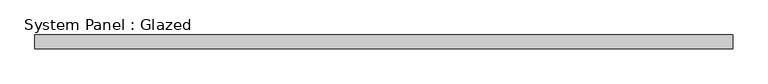
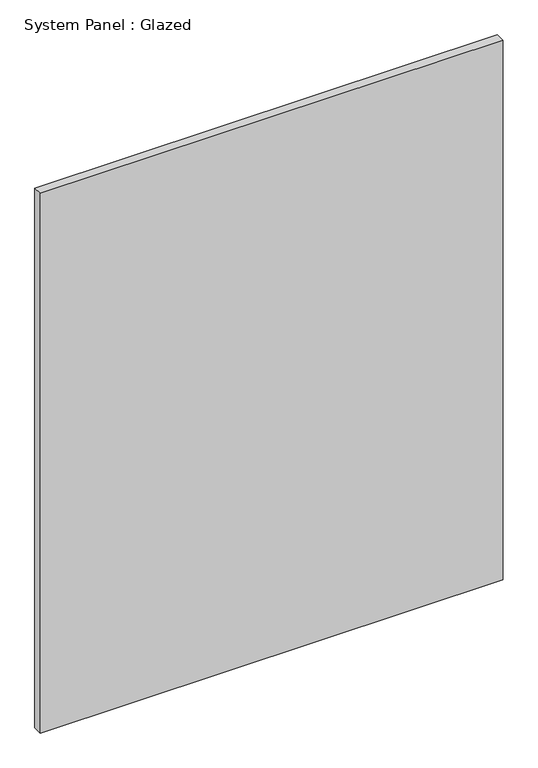
"""IFC4 building model written with IfcOpenShell, lengths in millimetres: plate geometry, System Panel : Glazed."""

from ifc_helpers import new_model, si_unit, origin, origin_with_axes, place, context, project, spatial, polyline, outline, extrude, source, transform, mapped, element, save


def system_panel_glazed_79b5039f(model_context):
    return source(origin(), model_context, "Body", "SweptSolid", [
        extrude(outline(polyline([(633.0541355, 24.5), (-633.0541355, 24.5), (-633.0541355, 49.5), (633.0541355, 49.5), (633.0541355, 24.5)])), origin_with_axes(), (0.0, 0.0, 1.0), 1560.0991456),
    ])


if __name__ == "__main__":
    model = new_model("IFC4")
    model_context = context("Model", 3, world=origin())
    ifc_project = project(units=[si_unit("LENGTHUNIT", "METRE", prefix="MILLI")], contexts=[model_context])
    site = spatial("IfcSite", under=ifc_project)
    building = spatial("IfcBuilding", under=site)
    placement = place(None, origin())
    system_panel_glazed_shape = system_panel_glazed_79b5039f(model_context)
    element("IfcPlate", 1, ObjectType="System Panel : Glazed", at=placement, inside=building, context=model_context, shape_type="MappedRepresentation", body=[
        mapped(system_panel_glazed_shape, transform((0.0, 0.0, 0.0), x_axis=(1.0, 0.0, 0.0), y_axis=(0.0, 1.0, 0.0), z_axis=(0.0, 0.0, 1.0))),
    ])
    save(model, "model.ifc")

# Revit data of these elements
# Type "System Panel : Glazed"
#   Construction Type Id = "GSP4R"
#   Analytic Construction = "1/8 in Pilkington single glazing"
#   Visual Light Transmittance = 0.9
#   Solar Heat Gain Coefficient = 0.86
#   Heat Transfer Coefficient (U) = 6.7069 W/(m²·K)
#   Define Thermal Properties by = 1
# Element 1 (IfcPlate, "System Panel : Glazed")
#   Materials on its faces: "Glass"
# Materials
#   "Glass": class "Glass", colour RGB 0 128 192, transparency 0.9, Description = "Soda Lime Glass", Cost = 0
